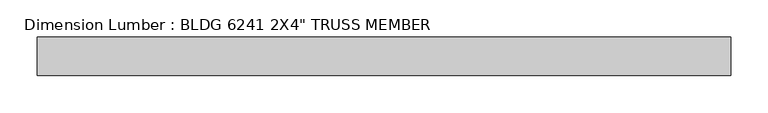
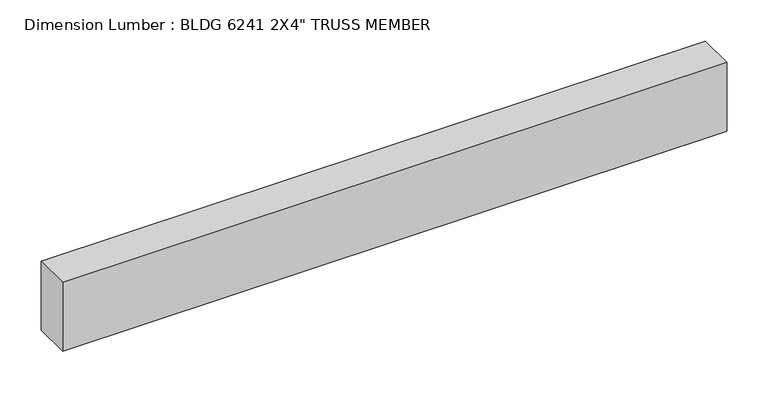
"""IFC4 building model written with IfcOpenShell, lengths in millimetres: beam geometry."""

from ifc_helpers import new_model, si_unit, frame, origin, place, context, project, spatial, polyline, outline, extrude, source, transform, mapped, element, save


def beam_0fe92c09(model_context):
    return source(origin(), model_context, "Body", "SweptSolid", [
        extrude(outline(polyline([(431.690501, 25.4), (431.690501, -25.4), (-492.3733183, -25.4), (-492.3733183, 25.4), (431.690501, 25.4)])), frame((0.0, 0.0, -50.8), z_axis=(0.0, 0.0, 1.0), x_axis=(1.0, 0.0, 0.0)), (0.0, 0.0, 1.0), 101.6),
    ])


if __name__ == "__main__":
    model = new_model("IFC4")
    model_context = context("Model", 3, world=origin())
    ifc_project = project(units=[si_unit("LENGTHUNIT", "METRE", prefix="MILLI")], contexts=[model_context])
    site = spatial("IfcSite", under=ifc_project)
    building = spatial("IfcBuilding", under=site)
    placement = place(None, origin())
    beam_shape = beam_0fe92c09(model_context)
    element("IfcBeam", 1, ObjectType="Dimension Lumber : BLDG 6241 2X4\" TRUSS MEMBER", at=placement, inside=building, context=model_context, shape_type="MappedRepresentation", body=[
        mapped(beam_shape, transform((0.0, 0.0, 0.0), x_axis=(1.0, 0.0, 0.0), y_axis=(0.0, 1.0, 0.0), z_axis=(0.0, 0.0, 1.0))),
    ])
    save(model, "model.ifc")

# Revit data of these elements
# Type "Dimension Lumber : BLDG 6241 2X4\" TRUSS MEMBER"
#   Assembly Code = "B10"
#   A = 0.273472 SF
#   Length [instance default] = 5' - 0"
#   b = 0' - 2"
#   d = 0' - 4"
#   Structural Material [instance default] = Softwood, Lumber
# Element 1 (IfcBeam, "Dimension Lumber : BLDG 6241 2X4\" TRUSS MEMBER")
#   Materials on its faces: "Softwood, Lumber"
# Materials
#   "Softwood, Lumber": class "Wood", colour RGB 223 192 134, transparency 0, Description = "Pinus Echinata", Cost = 0
